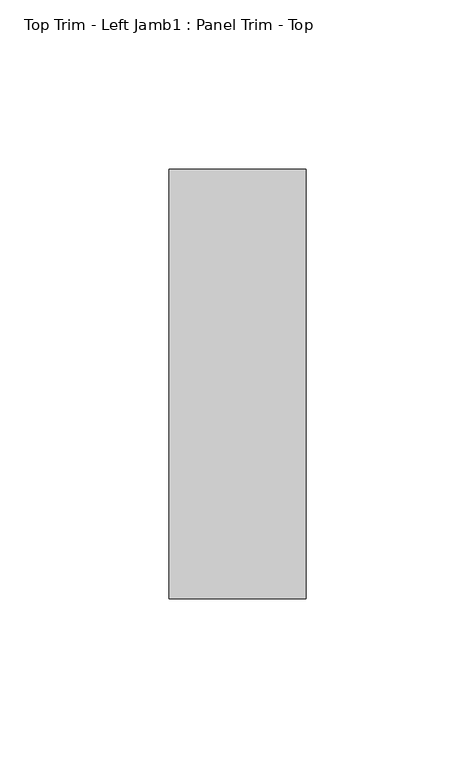
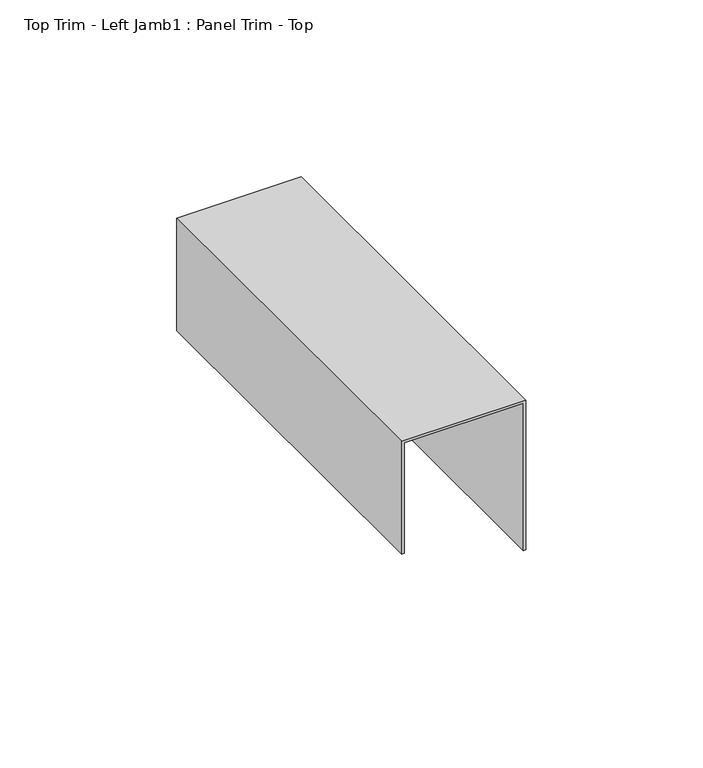
"""IFC4 building model written with IfcOpenShell, lengths in millimetres: proxy geometry, Top Trim - Left Jamb1 : Panel Trim - Top."""

from ifc_helpers import new_model, si_unit, frame, origin, place, context, project, spatial, polyline, outline, extrude, source, transform, mapped, element, save


def top_trim_left_jamb1_panel_trim_top_a1816676(model_context):
    return source(origin(), model_context, "Body", "SweptSolid", [
        extrude(outline(polyline([(2438.4, 587327.0060739), (2438.4, 587365.8934739), (2387.6, 587365.8934739), (2387.6, 587366.6808739), (2439.19375, 587366.6808739), (2439.19375, 587326.2186739), (2400.3, 587326.2186739), (2400.3, 587327.0060739), (2438.4, 587327.0060739)])), frame((0.0, -536420.7663841, 0.0), z_axis=(0.0, 1.0, 0.0), x_axis=(0.0, 0.0, 1.0)), (0.0, 0.0, 1.0), 127.0),
    ])


if __name__ == "__main__":
    model = new_model("IFC4")
    model_context = context("Model", 3, world=origin())
    ifc_project = project(units=[si_unit("LENGTHUNIT", "METRE", prefix="MILLI")], contexts=[model_context])
    site = spatial("IfcSite", under=ifc_project)
    building = spatial("IfcBuilding", under=site)
    placement = place(None, origin())
    top_trim_left_jamb1_panel_trim_top_shape = top_trim_left_jamb1_panel_trim_top_a1816676(model_context)
    element("IfcBuildingElementProxy", 1, Name="Top Trim - Left Jamb1 : Panel Trim - Top", ObjectType="Top Trim - Left Jamb1 : Panel Trim - Top", at=placement, inside=building, context=model_context, shape_type="MappedRepresentation", body=[
        mapped(top_trim_left_jamb1_panel_trim_top_shape, transform((0.0, 0.0, 0.0), x_axis=(1.0, 0.0, 0.0), y_axis=(0.0, 1.0, 0.0), z_axis=(0.0, 0.0, 1.0))),
    ])
    save(model, "model.ifc")

# Revit data of these elements
# Element 1 (IfcBuildingElementProxy, "Top Trim - Left Jamb1 : Panel Trim - Top")
#   Materials on its faces: "EDGE TRIM BY MTL PANEL MFR."
# Materials
#   "EDGE TRIM BY MTL PANEL MFR.": class "Generic", colour RGB 239 242 240, transparency 0, Cost = 0
